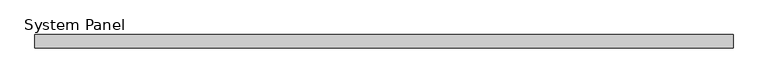
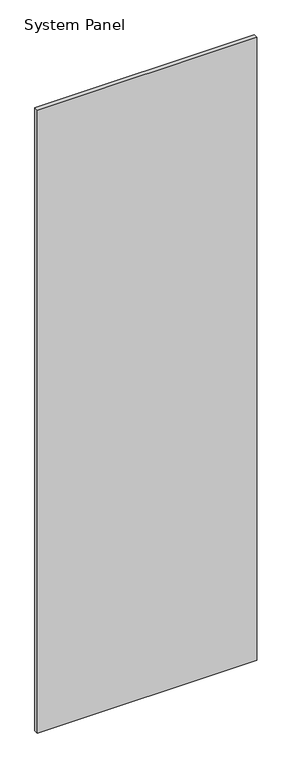
"""IFC4 building model written with IfcOpenShell, lengths in millimetres: plate geometry, System Panel : WWm-Glass-20mm-10mmOffset."""

import ifcopenshell
import ifcopenshell.guid

model = None  # the IFC model being written
_history = None  # IfcOwnerHistory: only IFC2X3 demands one
_inside = {}  # id of a spatial element -> (the spatial element, [elements in it])
_under = {}  # id of a project, library or spatial element -> (it, [spatial elements below it])
_declared = {}  # id of a project -> (the project, [libraries it declares])
_typed = {}  # id of a type object -> (the type object, [elements of that type])
_made_of = {}  # id of a material, layer set ... -> (it, [elements and type objects made of it])


def new_model(schema):
    """Start an empty IFC model of exactly this schema.

    Asked for "IFC4X3", IfcOpenShell would pick the latest addendum, in which some entities
    have other attributes; the version numbers below select the first issue.
    IFC2X3 requires an IfcOwnerHistory on every rooted entity: one is made here for all.
    """
    global model, _history
    if schema == "IFC4X3":
        model = ifcopenshell.file(schema_version=(4, 3, 0, 0))
    else:
        model = ifcopenshell.file(schema=schema)
    _inside.clear()
    _under.clear()
    _declared.clear()
    _typed.clear()
    _made_of.clear()
    _history = None
    if model.schema == "IFC2X3":
        org = make("IfcOrganization", Name="unknown")
        user = make(
            "IfcPersonAndOrganization",
            ThePerson=make("IfcPerson", FamilyName="unknown"),
            TheOrganization=org,
        )
        app = make(
            "IfcApplication",
            ApplicationDeveloper=org,
            Version="unknown",
            ApplicationFullName="unknown",
            ApplicationIdentifier="unknown",
        )
        _history = make(
            "IfcOwnerHistory",
            OwningUser=user,
            OwningApplication=app,
            ChangeAction="ADDED",
            CreationDate=0,
        )
    return model


def make(cls, **values):
    """One entity of the class cls with the attributes given. An attribute that is None is left unset."""
    return model.create_entity(
        cls, **{name: value for name, value in values.items() if value is not None}
    )


def rooted(cls, **values):
    """An entity with a GlobalId (a new one), such as an element, a storey or a relation."""
    return make(cls, GlobalId=ifcopenshell.guid.new(), OwnerHistory=_history, **values)


def si_unit(unit_type, name, prefix=None):
    """IfcSIUnit, for example si_unit("LENGTHUNIT", "METRE", prefix="MILLI")."""
    return make("IfcSIUnit", UnitType=unit_type, Prefix=prefix, Name=name)


def assignment(units):
    """IfcUnitAssignment: the units of a project."""
    return None if units is None else make("IfcUnitAssignment", Units=units)


def point(xyz):
    """IfcCartesianPoint."""
    return None if xyz is None else make("IfcCartesianPoint", Coordinates=xyz)


def direction(xyz):
    """IfcDirection."""
    return None if xyz is None else make("IfcDirection", DirectionRatios=xyz)


def frame(location, z_axis=None, x_axis=None):
    """IfcAxis2Placement3D, a coordinate frame: its origin and axes. An axis left out is left unset."""
    return make(
        "IfcAxis2Placement3D",
        Location=point(location),
        Axis=direction(z_axis),
        RefDirection=direction(x_axis),
    )


def origin():
    """The frame at (0, 0, 0) with its axes left unset."""
    return frame((0.0, 0.0, 0.0))


def origin_with_axes():
    """The frame at (0, 0, 0) with the z axis (0, 0, 1) and the x axis (1, 0, 0) written out."""
    return frame((0.0, 0.0, 0.0), z_axis=(0.0, 0.0, 1.0), x_axis=(1.0, 0.0, 0.0))


def place(relative_to, where):
    """IfcLocalPlacement: puts the frame where relative to a parent placement (None: the world)."""
    return make(
        "IfcLocalPlacement", PlacementRelTo=relative_to, RelativePlacement=where
    )


def context(
    kind, dimensions, precision=None, world=None, true_north=None, identifier=None
):
    """IfcGeometricRepresentationContext, for example the 3D "Model" context."""
    return make(
        "IfcGeometricRepresentationContext",
        ContextIdentifier=identifier,
        ContextType=kind,
        CoordinateSpaceDimension=dimensions,
        Precision=precision,
        WorldCoordinateSystem=world,
        TrueNorth=true_north,
    )


def project(units=None, contexts=None):
    """IfcProject with its units and contexts."""
    return rooted(
        "IfcProject",
        Name="project",
        RepresentationContexts=contexts,
        UnitsInContext=assignment(units),
    )


def spatial(cls, under=None, at=None, **own):
    """A site, building, storey or space (cls), placed at a placement, below another one or the project."""
    s = rooted(cls, ObjectPlacement=at, **own)
    if under is not None:
        _under.setdefault(under.id(), (under, []))[1].append(s)
    return s


def polyline(points):
    """IfcPolyline through the points."""
    return make("IfcPolyline", Points=[point(p) for p in points])


def outline(outer, holes=None, kind="AREA"):
    """IfcArbitraryClosedProfileDef: a profile drawn as a closed curve; with holes, ...WithVoids."""
    if holes is None:
        return make("IfcArbitraryClosedProfileDef", ProfileType=kind, OuterCurve=outer)
    return make(
        "IfcArbitraryProfileDefWithVoids",
        ProfileType=kind,
        OuterCurve=outer,
        InnerCurves=holes,
    )


def extrude(swept, where, along, depth):
    """IfcExtrudedAreaSolid: the profile swept, set in the frame where, extruded along a direction by depth."""
    return make(
        "IfcExtrudedAreaSolid",
        SweptArea=swept,
        Position=where,
        ExtrudedDirection=direction(along),
        Depth=depth,
    )


def shape(context_of_items, identifier, shape_type, items):
    """IfcShapeRepresentation: the items that make up one representation, for example the "Body"."""
    return make(
        "IfcShapeRepresentation",
        ContextOfItems=context_of_items,
        RepresentationIdentifier=identifier,
        RepresentationType=shape_type,
        Items=items,
    )


def source(mapping_origin, context_of_items, identifier, shape_type, items):
    """IfcRepresentationMap: a shape defined once, which mapped items show again and again."""
    return make(
        "IfcRepresentationMap",
        MappingOrigin=mapping_origin,
        MappedRepresentation=shape(context_of_items, identifier, shape_type, items),
    )


def transform(
    local_origin,
    x_axis=None,
    y_axis=None,
    z_axis=None,
    scale=None,
    scale2=None,
    scale3=None,
    uniform=True,
):
    """IfcCartesianTransformationOperator3D, or its non-uniform kind. x_axis, y_axis, z_axis: its Axis1, 2, 3."""
    if uniform:
        return make(
            "IfcCartesianTransformationOperator3D",
            Axis1=direction(x_axis),
            Axis2=direction(y_axis),
            LocalOrigin=point(local_origin),
            Scale=scale,
            Axis3=direction(z_axis),
        )
    return make(
        "IfcCartesianTransformationOperator3DnonUniform",
        Axis1=direction(x_axis),
        Axis2=direction(y_axis),
        LocalOrigin=point(local_origin),
        Scale=scale,
        Axis3=direction(z_axis),
        Scale2=scale2,
        Scale3=scale3,
    )


def mapped(mapping_source, mapping_target):
    """IfcMappedItem: shows the shape of a source again, moved by a transform."""
    return make(
        "IfcMappedItem", MappingSource=mapping_source, MappingTarget=mapping_target
    )


def made_of(thing, what):
    """Note that an element or type object is made of a material, layer set ...; save() writes the relation."""
    if what is not None:
        _made_of.setdefault(what.id(), (what, []))[1].append(thing)
    return thing


def element(
    cls,
    number,
    at=None,
    inside=None,
    cuts=None,
    type_object=None,
    material=None,
    context=None,
    identifier="Body",
    shape_type=None,
    held_by="IfcProductDefinitionShape",
    body=None,
    shapes=None,
    **own,
):
    """One element of the class cls, such as IfcWall. Its Tag is "e" and its number.

    at: its placement. inside: the storey or other place that contains it. cuts: it is an
    opening in that element (IfcRelVoidsElement). A single representation is given by context,
    identifier, shape_type and body (its items); several are given by shapes. held_by: the class
    of the entity that holds the representations. save() writes the other relations.
    """
    e = rooted(cls, Tag="e%d" % number, ObjectPlacement=at, **own)
    if body is not None:
        shapes = [shape(context, identifier, shape_type, body)]
    if shapes is not None:
        e.Representation = make(held_by, Representations=shapes)
    if inside is not None:
        _inside.setdefault(inside.id(), (inside, []))[1].append(e)
    if cuts is not None:
        rooted(
            "IfcRelVoidsElement", RelatingBuildingElement=cuts, RelatedOpeningElement=e
        )
    if type_object is not None:
        _typed.setdefault(type_object.id(), (type_object, []))[1].append(e)
    return made_of(e, material)


def aggregate(whole, parts):
    """IfcRelAggregates: a whole, such as a stair, and the parts it consists of."""
    return rooted("IfcRelAggregates", RelatingObject=whole, RelatedObjects=parts)


def save(model, path):
    """Write the relations noted so far, then the file.

    IfcRelAggregates (storeys below a building ...), IfcRelContainedInSpatialStructure (elements
    in a storey), IfcRelDefinesByType, IfcRelAssociatesMaterial and IfcRelDeclares: one each for
    every whole, place, type object, material and project.
    """
    for whole, parts in _under.values():
        aggregate(whole, parts)
    for where, things in _inside.values():
        rooted(
            "IfcRelContainedInSpatialStructure",
            RelatedElements=things,
            RelatingStructure=where,
        )
    for kind, things in _typed.values():
        rooted("IfcRelDefinesByType", RelatedObjects=things, RelatingType=kind)
    for what, things in _made_of.values():
        rooted("IfcRelAssociatesMaterial", RelatedObjects=things, RelatingMaterial=what)
    for by, libraries in _declared.values():
        rooted("IfcRelDeclares", RelatingContext=by, RelatedDefinitions=libraries)
    model.write(path)


def system_panel_725a6024(model_context):
    return source(origin(), model_context, "Body", "SweptSolid", [
        extrude(outline(polyline([(525.0, 0.0), (-525.0, 0.0), (-525.0, 20.0), (525.0, 20.0), (525.0, 0.0)])), origin_with_axes(), (0.0, 0.0, 1.0), 3150.0),
    ])


if __name__ == "__main__":
    model = new_model("IFC4")
    model_context = context("Model", 3, world=origin())
    ifc_project = project(units=[si_unit("LENGTHUNIT", "METRE", prefix="MILLI")], contexts=[model_context])
    site = spatial("IfcSite", under=ifc_project)
    building = spatial("IfcBuilding", under=site)
    placement = place(None, origin())
    system_panel_shape = system_panel_725a6024(model_context)
    element("IfcPlate", 1, ObjectType="System Panel : WWm-Glass-20mm-10mmOffset", at=placement, inside=building, context=model_context, shape_type="MappedRepresentation", body=[
        mapped(system_panel_shape, transform((0.0, 0.0, 0.0), x_axis=(1.0, 0.0, 0.0), y_axis=(0.0, 1.0, 0.0), z_axis=(0.0, 0.0, 1.0))),
    ])
    save(model, "model.ifc")

# Revit data of these elements
# Type "System Panel : WWm-Glass-20mm-10mmOffset"
#   Finish = ""
# Element 1 (IfcPlate, "System Panel : WWm-Glass-20mm-10mmOffset")
#   Materials on its faces: "WW-EC-GL-Storefront"
# Materials
#   "WW-EC-GL-Storefront": class "Glass", colour RGB 236 240 239, transparency 0.85, Description = "Storefront Glass", Cost = 0
